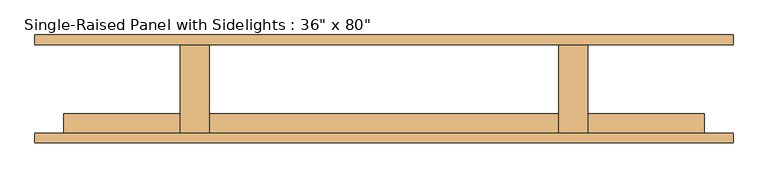
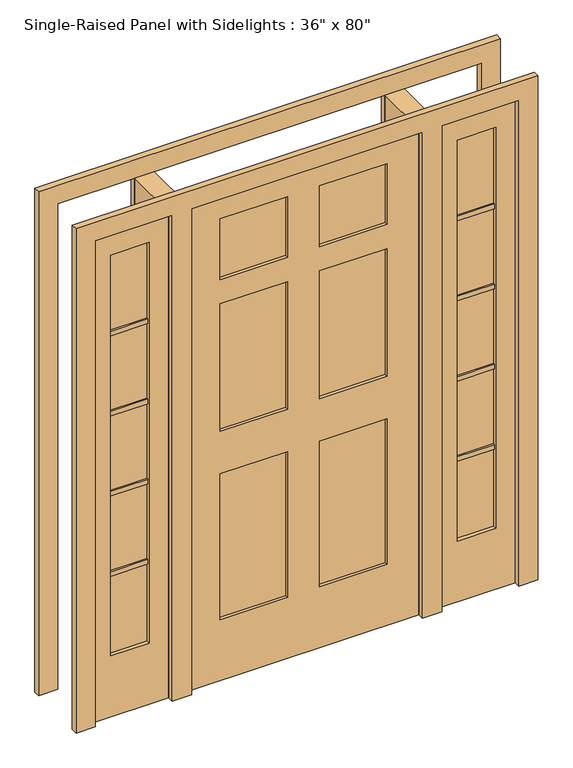
"""IFC4 building model written with IfcOpenShell, lengths in millimetres: door geometry."""

import ifcopenshell
import ifcopenshell.guid

model = None  # the IFC model being written
_history = None  # IfcOwnerHistory: only IFC2X3 demands one
_inside = {}  # id of a spatial element -> (the spatial element, [elements in it])
_under = {}  # id of a project, library or spatial element -> (it, [spatial elements below it])
_declared = {}  # id of a project -> (the project, [libraries it declares])
_typed = {}  # id of a type object -> (the type object, [elements of that type])
_made_of = {}  # id of a material, layer set ... -> (it, [elements and type objects made of it])


def new_model(schema):
    """Start an empty IFC model of exactly this schema.

    Asked for "IFC4X3", IfcOpenShell would pick the latest addendum, in which some entities
    have other attributes; the version numbers below select the first issue.
    IFC2X3 requires an IfcOwnerHistory on every rooted entity: one is made here for all.
    """
    global model, _history
    if schema == "IFC4X3":
        model = ifcopenshell.file(schema_version=(4, 3, 0, 0))
    else:
        model = ifcopenshell.file(schema=schema)
    _inside.clear()
    _under.clear()
    _declared.clear()
    _typed.clear()
    _made_of.clear()
    _history = None
    if model.schema == "IFC2X3":
        org = make("IfcOrganization", Name="unknown")
        user = make(
            "IfcPersonAndOrganization",
            ThePerson=make("IfcPerson", FamilyName="unknown"),
            TheOrganization=org,
        )
        app = make(
            "IfcApplication",
            ApplicationDeveloper=org,
            Version="unknown",
            ApplicationFullName="unknown",
            ApplicationIdentifier="unknown",
        )
        _history = make(
            "IfcOwnerHistory",
            OwningUser=user,
            OwningApplication=app,
            ChangeAction="ADDED",
            CreationDate=0,
        )
    return model


def make(cls, **values):
    """One entity of the class cls with the attributes given. An attribute that is None is left unset."""
    return model.create_entity(
        cls, **{name: value for name, value in values.items() if value is not None}
    )


def rooted(cls, **values):
    """An entity with a GlobalId (a new one), such as an element, a storey or a relation."""
    return make(cls, GlobalId=ifcopenshell.guid.new(), OwnerHistory=_history, **values)


def si_unit(unit_type, name, prefix=None):
    """IfcSIUnit, for example si_unit("LENGTHUNIT", "METRE", prefix="MILLI")."""
    return make("IfcSIUnit", UnitType=unit_type, Prefix=prefix, Name=name)


def assignment(units):
    """IfcUnitAssignment: the units of a project."""
    return None if units is None else make("IfcUnitAssignment", Units=units)


def point(xyz):
    """IfcCartesianPoint."""
    return None if xyz is None else make("IfcCartesianPoint", Coordinates=xyz)


def direction(xyz):
    """IfcDirection."""
    return None if xyz is None else make("IfcDirection", DirectionRatios=xyz)


def frame(location, z_axis=None, x_axis=None):
    """IfcAxis2Placement3D, a coordinate frame: its origin and axes. An axis left out is left unset."""
    return make(
        "IfcAxis2Placement3D",
        Location=point(location),
        Axis=direction(z_axis),
        RefDirection=direction(x_axis),
    )


def origin():
    """The frame at (0, 0, 0) with its axes left unset."""
    return frame((0.0, 0.0, 0.0))


def origin_with_axes():
    """The frame at (0, 0, 0) with the z axis (0, 0, 1) and the x axis (1, 0, 0) written out."""
    return frame((0.0, 0.0, 0.0), z_axis=(0.0, 0.0, 1.0), x_axis=(1.0, 0.0, 0.0))


def place(relative_to, where):
    """IfcLocalPlacement: puts the frame where relative to a parent placement (None: the world)."""
    return make(
        "IfcLocalPlacement", PlacementRelTo=relative_to, RelativePlacement=where
    )


def context(
    kind, dimensions, precision=None, world=None, true_north=None, identifier=None
):
    """IfcGeometricRepresentationContext, for example the 3D "Model" context."""
    return make(
        "IfcGeometricRepresentationContext",
        ContextIdentifier=identifier,
        ContextType=kind,
        CoordinateSpaceDimension=dimensions,
        Precision=precision,
        WorldCoordinateSystem=world,
        TrueNorth=true_north,
    )


def project(units=None, contexts=None):
    """IfcProject with its units and contexts."""
    return rooted(
        "IfcProject",
        Name="project",
        RepresentationContexts=contexts,
        UnitsInContext=assignment(units),
    )


def spatial(cls, under=None, at=None, **own):
    """A site, building, storey or space (cls), placed at a placement, below another one or the project."""
    s = rooted(cls, ObjectPlacement=at, **own)
    if under is not None:
        _under.setdefault(under.id(), (under, []))[1].append(s)
    return s


def polyline(points):
    """IfcPolyline through the points."""
    return make("IfcPolyline", Points=[point(p) for p in points])


def outline(outer, holes=None, kind="AREA"):
    """IfcArbitraryClosedProfileDef: a profile drawn as a closed curve; with holes, ...WithVoids."""
    if holes is None:
        return make("IfcArbitraryClosedProfileDef", ProfileType=kind, OuterCurve=outer)
    return make(
        "IfcArbitraryProfileDefWithVoids",
        ProfileType=kind,
        OuterCurve=outer,
        InnerCurves=holes,
    )


def extrude(swept, where, along, depth):
    """IfcExtrudedAreaSolid: the profile swept, set in the frame where, extruded along a direction by depth."""
    return make(
        "IfcExtrudedAreaSolid",
        SweptArea=swept,
        Position=where,
        ExtrudedDirection=direction(along),
        Depth=depth,
    )


def shape(context_of_items, identifier, shape_type, items):
    """IfcShapeRepresentation: the items that make up one representation, for example the "Body"."""
    return make(
        "IfcShapeRepresentation",
        ContextOfItems=context_of_items,
        RepresentationIdentifier=identifier,
        RepresentationType=shape_type,
        Items=items,
    )


def source(mapping_origin, context_of_items, identifier, shape_type, items):
    """IfcRepresentationMap: a shape defined once, which mapped items show again and again."""
    return make(
        "IfcRepresentationMap",
        MappingOrigin=mapping_origin,
        MappedRepresentation=shape(context_of_items, identifier, shape_type, items),
    )


def transform(
    local_origin,
    x_axis=None,
    y_axis=None,
    z_axis=None,
    scale=None,
    scale2=None,
    scale3=None,
    uniform=True,
):
    """IfcCartesianTransformationOperator3D, or its non-uniform kind. x_axis, y_axis, z_axis: its Axis1, 2, 3."""
    if uniform:
        return make(
            "IfcCartesianTransformationOperator3D",
            Axis1=direction(x_axis),
            Axis2=direction(y_axis),
            LocalOrigin=point(local_origin),
            Scale=scale,
            Axis3=direction(z_axis),
        )
    return make(
        "IfcCartesianTransformationOperator3DnonUniform",
        Axis1=direction(x_axis),
        Axis2=direction(y_axis),
        LocalOrigin=point(local_origin),
        Scale=scale,
        Axis3=direction(z_axis),
        Scale2=scale2,
        Scale3=scale3,
    )


def mapped(mapping_source, mapping_target):
    """IfcMappedItem: shows the shape of a source again, moved by a transform."""
    return make(
        "IfcMappedItem", MappingSource=mapping_source, MappingTarget=mapping_target
    )


def made_of(thing, what):
    """Note that an element or type object is made of a material, layer set ...; save() writes the relation."""
    if what is not None:
        _made_of.setdefault(what.id(), (what, []))[1].append(thing)
    return thing


def element(
    cls,
    number,
    at=None,
    inside=None,
    cuts=None,
    type_object=None,
    material=None,
    context=None,
    identifier="Body",
    shape_type=None,
    held_by="IfcProductDefinitionShape",
    body=None,
    shapes=None,
    **own,
):
    """One element of the class cls, such as IfcWall. Its Tag is "e" and its number.

    at: its placement. inside: the storey or other place that contains it. cuts: it is an
    opening in that element (IfcRelVoidsElement). A single representation is given by context,
    identifier, shape_type and body (its items); several are given by shapes. held_by: the class
    of the entity that holds the representations. save() writes the other relations.
    """
    e = rooted(cls, Tag="e%d" % number, ObjectPlacement=at, **own)
    if body is not None:
        shapes = [shape(context, identifier, shape_type, body)]
    if shapes is not None:
        e.Representation = make(held_by, Representations=shapes)
    if inside is not None:
        _inside.setdefault(inside.id(), (inside, []))[1].append(e)
    if cuts is not None:
        rooted(
            "IfcRelVoidsElement", RelatingBuildingElement=cuts, RelatedOpeningElement=e
        )
    if type_object is not None:
        _typed.setdefault(type_object.id(), (type_object, []))[1].append(e)
    return made_of(e, material)


def aggregate(whole, parts):
    """IfcRelAggregates: a whole, such as a stair, and the parts it consists of."""
    return rooted("IfcRelAggregates", RelatingObject=whole, RelatedObjects=parts)


def save(model, path):
    """Write the relations noted so far, then the file.

    IfcRelAggregates (storeys below a building ...), IfcRelContainedInSpatialStructure (elements
    in a storey), IfcRelDefinesByType, IfcRelAssociatesMaterial and IfcRelDeclares: one each for
    every whole, place, type object, material and project.
    """
    for whole, parts in _under.values():
        aggregate(whole, parts)
    for where, things in _inside.values():
        rooted(
            "IfcRelContainedInSpatialStructure",
            RelatedElements=things,
            RelatingStructure=where,
        )
    for kind, things in _typed.values():
        rooted("IfcRelDefinesByType", RelatedObjects=things, RelatingType=kind)
    for what, things in _made_of.values():
        rooted("IfcRelAssociatesMaterial", RelatedObjects=things, RelatingMaterial=what)
    for by, libraries in _declared.values():
        rooted("IfcRelDeclares", RelatingContext=by, RelatedDefinitions=libraries)
    model.write(path)


def door_2fa28ffd(model_context):
    return source(origin(), model_context, "Body", "SweptSolid", [
        extrude(outline(polyline([(762.0, -74.6125008), (762.0, -106.3625008), (609.6, -106.3625008), (609.6, -74.6125008), (762.0, -74.6125008)])), frame((0.0, 0.0, 579.755), z_axis=(0.0, 0.0, 1.0), x_axis=(1.0, 0.0, 0.0)), (0.0, 0.0, 1.0), 19.05),
        extrude(outline(polyline([(762.0, -74.6125008), (762.0, -106.3625008), (609.6, -106.3625008), (609.6, -74.6125008), (762.0, -74.6125008)])), frame((0.0, 0.0, 915.035), z_axis=(0.0, 0.0, 1.0), x_axis=(1.0, 0.0, 0.0)), (0.0, 0.0, 1.0), 19.05),
        extrude(outline(polyline([(762.0, -74.6125008), (762.0, -106.3625008), (609.6, -106.3625008), (609.6, -74.6125008), (762.0, -74.6125008)])), frame((0.0, 0.0, 1250.315), z_axis=(0.0, 0.0, 1.0), x_axis=(1.0, 0.0, 0.0)), (0.0, 0.0, 1.0), 19.05),
        extrude(outline(polyline([(762.0, -74.6125008), (762.0, -106.3625008), (609.6, -106.3625008), (609.6, -74.6125008), (762.0, -74.6125008)])), frame((0.0, 0.0, 1585.595), z_axis=(0.0, 0.0, 1.0), x_axis=(1.0, 0.0, 0.0)), (0.0, 0.0, 1.0), 19.05),
        extrude(outline(polyline([(-609.6, -74.6125008), (-609.6, -106.3625008), (-762.0, -106.3625008), (-762.0, -74.6125008), (-609.6, -74.6125008)])), frame((0.0, 0.0, 1585.595), z_axis=(0.0, 0.0, 1.0), x_axis=(1.0, 0.0, 0.0)), (0.0, 0.0, 1.0), 19.05),
        extrude(outline(polyline([(-609.6, -74.6125008), (-609.6, -106.3625008), (-762.0, -106.3625008), (-762.0, -74.6125008), (-609.6, -74.6125008)])), frame((0.0, 0.0, 1250.315), z_axis=(0.0, 0.0, 1.0), x_axis=(1.0, 0.0, 0.0)), (0.0, 0.0, 1.0), 19.05),
        extrude(outline(polyline([(-609.6, -74.6125008), (-609.6, -106.3625008), (-762.0, -106.3625008), (-762.0, -74.6125008), (-609.6, -74.6125008)])), frame((0.0, 0.0, 915.035), z_axis=(0.0, 0.0, 1.0), x_axis=(1.0, 0.0, 0.0)), (0.0, 0.0, 1.0), 19.05),
        extrude(outline(polyline([(-609.6, -74.6125008), (-609.6, -106.3625008), (-762.0, -106.3625008), (-762.0, -74.6125008), (-609.6, -74.6125008)])), frame((0.0, 0.0, 579.755), z_axis=(0.0, 0.0, 1.0), x_axis=(1.0, 0.0, 0.0)), (0.0, 0.0, 1.0), 19.05),
        extrude(outline(polyline([(762.0, -80.9625008), (762.0, -100.0125008), (609.6, -100.0125008), (609.6, -80.9625008), (762.0, -80.9625008)])), frame((0.0, 0.0, 254.0), z_axis=(0.0, 0.0, 1.0), x_axis=(1.0, 0.0, 0.0)), (0.0, 0.0, 1.0), 1676.4),
        extrude(outline(polyline([(-609.6, -80.9625008), (-609.6, -100.0125008), (-762.0, -100.0125008), (-762.0, -80.9625008), (-609.6, -80.9625008)])), frame((0.0, 0.0, 254.0), z_axis=(0.0, 0.0, 1.0), x_axis=(1.0, 0.0, 0.0)), (0.0, 0.0, 1.0), 1676.4),
        extrude(outline(polyline([(-457.2, 115.8875008), (-457.2, -115.8875008), (-533.4, -115.8875008), (-533.4, 115.8875008), (-457.2, 115.8875008)])), origin_with_axes(), (0.0, 0.0, 1.0), 2032.0),
        extrude(outline(polyline([(533.4, 115.8875008), (533.4, -115.8875008), (457.2, -115.8875008), (457.2, 115.8875008), (533.4, 115.8875008)])), origin_with_axes(), (0.0, 0.0, 1.0), 2032.0),
        extrude(outline(polyline([(2032.0, -533.4), (2032.0, -838.2), (0.0, -838.2), (0.0, -533.4), (2032.0, -533.4)]), holes=[polyline([(1930.4, -609.6), (254.0, -609.6), (254.0, -762.0), (1930.4, -762.0), (1930.4, -609.6)])]), frame((0.0, -115.8875008, 0.0), z_axis=(0.0, 1.0, 0.0), x_axis=(0.0, 0.0, 1.0)), (0.0, 0.0, 1.0), 50.8),
        extrude(outline(polyline([(0.0, 533.4), (0.0, 838.2), (2032.0, 838.2), (2032.0, 533.4), (0.0, 533.4)]), holes=[polyline([(1930.4, 762.0), (254.0, 762.0), (254.0, 609.6), (1930.4, 609.6), (1930.4, 762.0)])]), frame((0.0, -115.8875008, 0.0), z_axis=(0.0, 1.0, 0.0), x_axis=(0.0, 0.0, 1.0)), (0.0, 0.0, 1.0), 50.8),
        extrude(outline(polyline([(0.0, -914.4), (0.0, -838.2), (2032.0, -838.2), (2032.0, -533.4), (0.0, -533.4), (0.0, -457.2), (2032.0, -457.2), (2032.0, 457.2), (0.0, 457.2), (0.0, 533.4), (2032.0, 533.4), (2032.0, 838.2), (0.0, 838.2), (0.0, 914.4), (2108.2, 914.4), (2108.2, -914.4), (0.0, -914.4)])), frame((0.0, 115.8875008, 0.0), z_axis=(0.0, 1.0, 0.0), x_axis=(0.0, 0.0, 1.0)), (0.0, 0.0, 1.0), 25.4),
        extrude(outline(polyline([(0.0, 914.4), (2108.2, 914.4), (2108.2, -914.4), (0.0, -914.4), (0.0, -838.2), (2032.0, -838.2), (2032.0, -533.4), (0.0, -533.4), (0.0, -457.2), (2032.0, -457.2), (2032.0, 457.2), (0.0, 457.2), (0.0, 533.4), (2032.0, 533.4), (2032.0, 838.2), (0.0, 838.2), (0.0, 914.4)])), frame((0.0, -141.2875008, 0.0), z_axis=(0.0, 1.0, 0.0), x_axis=(0.0, 0.0, 1.0)), (0.0, 0.0, 1.0), 25.4),
        extrude(outline(polyline([(-63.5, -77.7875008), (-63.5, -103.1875008), (-330.2, -103.1875008), (-330.2, -77.7875008), (-63.5, -77.7875008)])), frame((0.0, 0.0, 1676.4), z_axis=(0.0, 0.0, 1.0), x_axis=(1.0, 0.0, 0.0)), (0.0, 0.0, 1.0), 254.0),
        extrude(outline(polyline([(330.2, -77.7875008), (330.2, -103.1875008), (63.5, -103.1875008), (63.5, -77.7875008), (330.2, -77.7875008)])), frame((0.0, 0.0, 1676.4), z_axis=(0.0, 0.0, 1.0), x_axis=(1.0, 0.0, 0.0)), (0.0, 0.0, 1.0), 254.0),
        extrude(outline(polyline([(-63.5, -77.7875008), (-63.5, -103.1875008), (-330.2, -103.1875008), (-330.2, -77.7875008), (-63.5, -77.7875008)])), frame((0.0, 0.0, 1041.4), z_axis=(0.0, 0.0, 1.0), x_axis=(1.0, 0.0, 0.0)), (0.0, 0.0, 1.0), 533.4),
        extrude(outline(polyline([(330.2, -77.7875008), (330.2, -103.1875008), (63.5, -103.1875008), (63.5, -77.7875008), (330.2, -77.7875008)])), frame((0.0, 0.0, 1041.4), z_axis=(0.0, 0.0, 1.0), x_axis=(1.0, 0.0, 0.0)), (0.0, 0.0, 1.0), 533.4),
        extrude(outline(polyline([(-63.5, -77.7875008), (-63.5, -103.1875008), (-330.2, -103.1875008), (-330.2, -77.7875008), (-63.5, -77.7875008)])), frame((0.0, 0.0, 254.0), z_axis=(0.0, 0.0, 1.0), x_axis=(1.0, 0.0, 0.0)), (0.0, 0.0, 1.0), 609.6),
        extrude(outline(polyline([(330.2, -77.7875008), (330.2, -103.1875008), (63.5, -103.1875008), (63.5, -77.7875008), (330.2, -77.7875008)])), frame((0.0, 0.0, 254.0), z_axis=(0.0, 0.0, 1.0), x_axis=(1.0, 0.0, 0.0)), (0.0, 0.0, 1.0), 609.6),
        extrude(outline(polyline([(2032.0, 457.2), (2032.0, -457.2), (0.0, -457.2), (0.0, 457.2), (2032.0, 457.2)]), holes=[polyline([(1930.4, -63.5), (1676.4, -63.5), (1676.4, -330.2), (1930.4, -330.2), (1930.4, -63.5)]), polyline([(1930.4, 330.2), (1676.4, 330.2), (1676.4, 63.5), (1930.4, 63.5), (1930.4, 330.2)]), polyline([(1574.8, -63.5), (1041.4, -63.5), (1041.4, -330.2), (1574.8, -330.2), (1574.8, -63.5)]), polyline([(1574.8, 330.2), (1041.4, 330.2), (1041.4, 63.5), (1574.8, 63.5), (1574.8, 330.2)]), polyline([(863.6, -63.5), (254.0, -63.5), (254.0, -330.2), (863.6, -330.2), (863.6, -63.5)]), polyline([(863.6, 330.2), (254.0, 330.2), (254.0, 63.5), (863.6, 63.5), (863.6, 330.2)])]), frame((0.0, -115.8875008, 0.0), z_axis=(0.0, 1.0, 0.0), x_axis=(0.0, 0.0, 1.0)), (0.0, 0.0, 1.0), 50.8),
    ])


if __name__ == "__main__":
    model = new_model("IFC4")
    model_context = context("Model", 3, world=origin())
    ifc_project = project(units=[si_unit("LENGTHUNIT", "METRE", prefix="MILLI")], contexts=[model_context])
    site = spatial("IfcSite", under=ifc_project)
    building = spatial("IfcBuilding", under=site)
    placement = place(None, origin())
    door_shape = door_2fa28ffd(model_context)
    element("IfcDoor", 1, ObjectType="Single-Raised Panel with Sidelights : 36\" x 80\"", at=placement, inside=building, context=model_context, shape_type="MappedRepresentation", body=[
        mapped(door_shape, transform((0.0, 0.0, 0.0), x_axis=(1.0, 0.0, 0.0), y_axis=(0.0, 1.0, 0.0), z_axis=(0.0, 0.0, 1.0))),
    ])
    save(model, "model.ifc")

# Revit data of these elements
# Type "Single-Raised Panel with Sidelights : 36\" x 80\""
#   Type Mark = "70"
#   COBie.Type.CreatedBy = "doug.wood@us.ibm.com"
#   COBie.Type.CreatedOn = "2016-04-14T02:07:24"
#   COBie.Type.Name = "Doors_Single-Raised Panel with Sidelights_36\" x 80\"_70"
#   COBie.Type.Category = "23-30 10 00 : Doors"
#   COBie.Type.Description = "Single-Raised Panel with Sidelights_36\" x 80\""
#   COBie.Type.Manufacturer = ""
#   COBie.Type.ModelNumber = ""
#   Construction Type Id = "MDOOR"
#   Assembly Code = "C1020"
#   Analytic Construction = "Metal"
#   COBie.Type.ReplacementCost = 0
#   Thickness = 0' - 2"
#   Heat Transfer Coefficient (U) = 3.7021 W/(m²·K)
#   Height = 6' - 8"
#   Rail Width - Base = 0' - 10"
#   Rail Width - Center = 0' - 7"
#   Rail Width - Top = 0' - 4"
#   Sidelight Width = 1' - 0"
#   Stile Width = 0' - 5"
#   Trim Projection Ext = 0' - 1"
#   Trim Projection Int = 0' - 1"
#   Trim Width = 0' - 3"
#   Width = 3' - 0"
#   COBie.Type = no
#   Function = 1
#   Door Material = Door - Panel - White
#   Frame Material = Door - Frame - White
#   Visual Light Transmittance = 0
#   Solar Heat Gain Coefficient = 0
#   Wall Closure = (empty or 0)
# Element 1 (IfcDoor, "Single-Raised Panel with Sidelights : 36\" x 80\"")
#   Materials on its faces: "Door - Panel - White", "Door - Frame - White", "Glass"
# Materials
#   "Door - Panel - White": class "Wood", colour RGB 255 255 255, transparency 0, Cost = 0
#   "Door - Frame - White": class "Miscellaneous", colour RGB 255 255 255, transparency 0, Cost = 0
#   "Glass": class "Glass", colour RGB 0 128 192, transparency 0.75, Description = "Soda Lime Glass", Cost = 0
